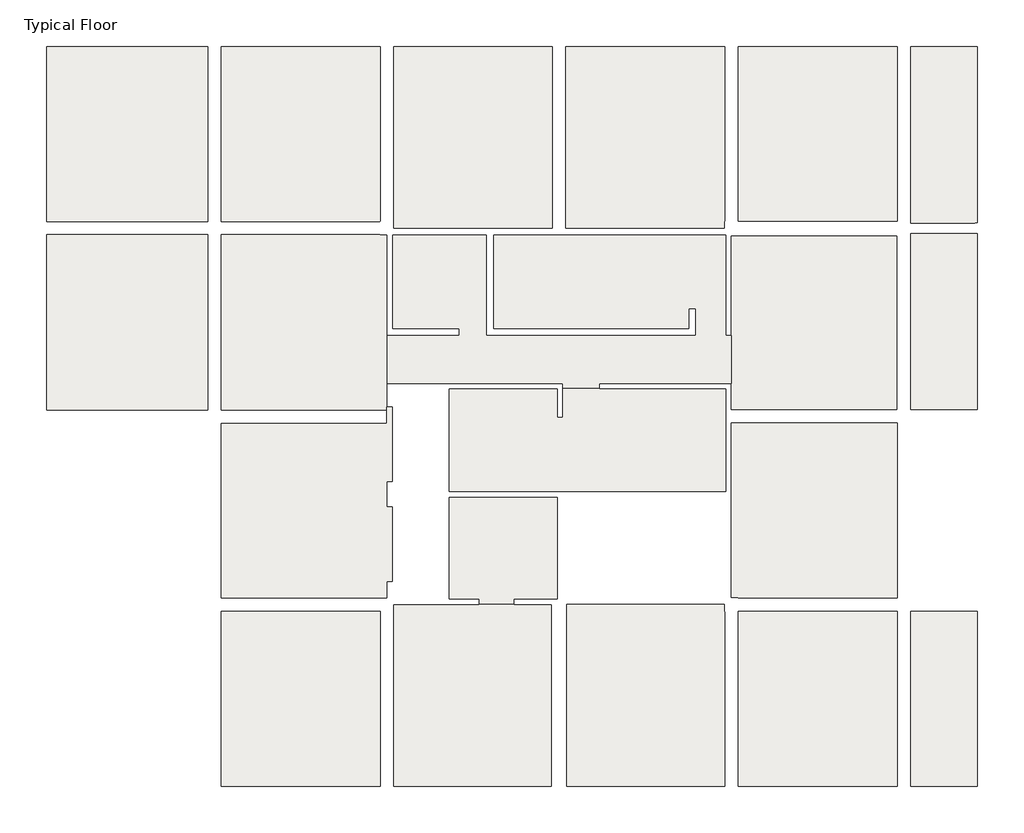
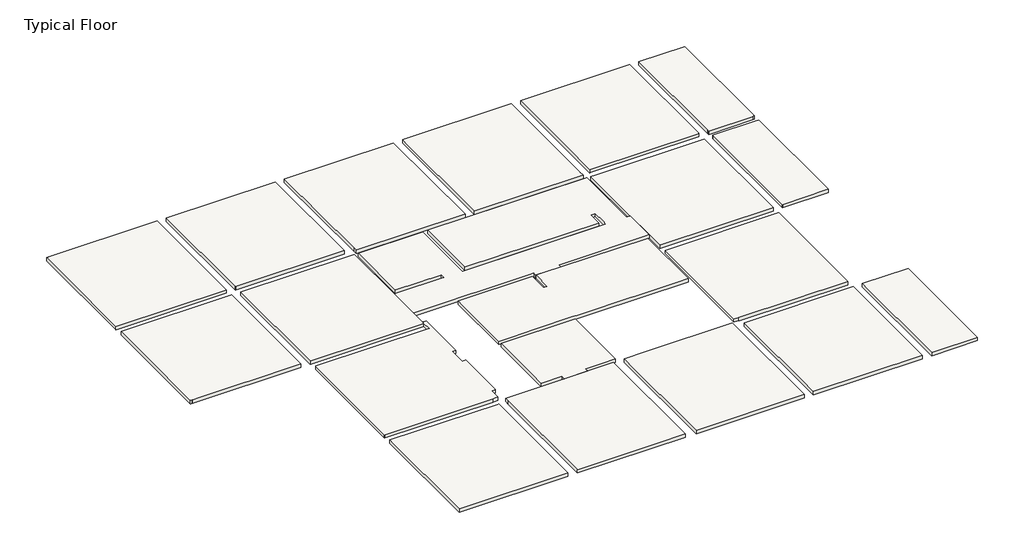
# One storey: 20 slabs.
"""IFC4 building model written with IfcOpenShell, lengths in millimetres."""

from ifc_helpers import new_model, si_unit, frame, origin, place, context, project, spatial, polyline, outline, extrude, faceted_brep, element, save

model = new_model("IFC4")

# Units and contexts
model_context = context("Model", 3, world=origin())
ifc_project = project(units=[si_unit("LENGTHUNIT", "METRE", prefix="MILLI")], contexts=[model_context])

# Site, building, storey
site = spatial("IfcSite", under=ifc_project)
building = spatial("IfcBuilding", under=site)
storey = spatial("IfcBuildingStorey", under=building, Name="Typical Floor", Elevation=4000.0)

# Slabs
placement = place(None, origin())
element("IfcSlab", 1, ObjectType="23", at=placement, inside=storey, context=model_context, shape_type="Brep", body=[
    faceted_brep([(8756.9599651, 6086.2983934, 3770.0), (-3356.6009397, 6086.2983934, 3770.0), (-3356.6009397, 10573.3383922, 3770.0), (1372.1290873, 10573.3383922, 3770.0), (1372.1290873, 9338.5905192, 3770.0), (1622.1290873, 9338.5905192, 3770.0), (1622.1290873, 10573.3383922, 3770.0), (1622.1290873, 10593.3383922, 3770.0), (3208.0390271, 10593.3383922, 3770.0), (3208.0390271, 10573.3383922, 3770.0), (8756.9599651, 10573.3383922, 3770.0), (-3356.6009397, 6086.2983934, 4000.0), (1378.3544453, 6086.2983934, 4000.0), (1628.3544453, 6086.2983934, 4000.0), (8756.9599651, 6086.2983934, 4000.0), (8756.9599651, 10573.3383922, 4000.0), (3208.0390271, 10573.3383922, 4000.0), (3208.0390271, 10593.3383922, 4000.0), (1622.1290873, 10593.3383922, 4000.0), (1622.1290873, 10573.3383922, 4000.0), (1622.1290873, 9338.5905192, 4000.0), (1372.1290873, 9338.5905192, 4000.0), (1372.1290873, 10573.3383922, 4000.0), (-3356.6009397, 10573.3383922, 4000.0)], [[[0, 1, 2, 3, 4, 5, 6, 7, 8, 9, 10]], [[11, 12, 13, 14, 15, 16, 17, 18, 19, 20, 21, 22, 23]], [[1, 0, 14, 13, 12, 11]], [[2, 1, 11, 23]], [[3, 2, 23, 22]], [[4, 3, 22, 21]], [[5, 4, 21, 20]], [[5, 20, 19, 18, 7, 6]], [[8, 7, 18, 17]], [[9, 8, 17, 16]], [[10, 9, 16, 15]], [[0, 10, 15, 14]]]),
])
element("IfcSlab", 2, ObjectType="23", at=placement, inside=storey, context=model_context, shape_type="Brep", body=[
    faceted_brep([(9298.3595467, 17938.0356779, 3770.0), (9298.3595467, 25592.9632364, 3770.0), (9303.3595467, 25592.9632364, 3770.0), (9303.3595467, 25597.9632364, 3770.0), (16261.8802114, 25597.9632364, 3770.0), (16261.8802114, 25592.9632364, 3770.0), (16266.8802114, 25592.9632364, 3770.0), (16266.8802114, 17943.0356779, 3770.0), (16261.8802114, 17943.0356779, 3770.0), (16261.8802114, 17938.0356779, 3770.0), (9303.3595467, 17938.0356779, 3770.0), (9298.3595467, 25592.9632364, 4000.0), (9298.3595467, 17938.0356779, 4000.0), (9303.3595467, 17938.0356779, 4000.0), (16261.8802114, 17938.0356779, 4000.0), (16261.8802114, 17943.0356779, 4000.0), (16266.8802114, 17943.0356779, 4000.0), (16266.8802114, 25592.9632364, 4000.0), (16261.8802114, 25592.9632364, 4000.0), (16261.8802114, 25597.9632364, 4000.0), (9303.3595467, 25597.9632364, 4000.0), (9303.3595467, 25592.9632364, 4000.0)], [[[0, 1, 2, 3, 4, 5, 6, 7, 8, 9, 10]], [[11, 12, 13, 14, 15, 16, 17, 18, 19, 20, 21]], [[6, 17, 16, 7]], [[12, 0, 10, 9, 14, 13]], [[0, 12, 11, 1]], [[3, 20, 19, 4]], [[2, 21, 20, 3]], [[21, 2, 1, 11]], [[5, 18, 17, 6]], [[18, 5, 4, 19]], [[8, 15, 14, 9]], [[15, 8, 7, 16]]]),
])
element("IfcSlab", 3, ObjectType="23", at=placement, inside=storey, context=model_context, shape_type="Brep", body=[
    faceted_brep([(16861.8802114, 25597.9632364, 3770.0), (19788.3855721, 25597.9632364, 3770.0), (19788.3855721, 25592.9632364, 3770.0), (19788.3855721, 17886.6191558, 3770.0), (19778.3855721, 17886.6191558, 3770.0), (19678.3855721, 17886.6191558, 3770.0), (19678.3855721, 17863.0356779, 3770.0), (16861.8802114, 17863.0356779, 3770.0), (16861.8802114, 17936.6191558, 3770.0), (16861.8802114, 17943.0356779, 3770.0), (16856.8802114, 17943.0356779, 3770.0), (16856.8802114, 25592.9632364, 3770.0), (16861.8802114, 25592.9632364, 3770.0), (19788.3855721, 25597.9632364, 4000.0), (16861.8802114, 25597.9632364, 4000.0), (16861.8802114, 25592.9632364, 4000.0), (16856.8802114, 25592.9632364, 4000.0), (16856.8802114, 17943.0356779, 4000.0), (16861.8802114, 17943.0356779, 4000.0), (16861.8802114, 17863.0356779, 4000.0), (19678.3855721, 17863.0356779, 4000.0), (19678.3855721, 17886.6191558, 4000.0), (19788.3855721, 17886.6191558, 4000.0), (19788.3855721, 25592.9632364, 4000.0)], [[[0, 1, 2, 3, 4, 5, 6, 7, 8, 9, 10, 11, 12]], [[13, 14, 15, 16, 17, 18, 19, 20, 21, 22, 23]], [[1, 13, 23, 22, 3, 2]], [[19, 7, 6, 20]], [[16, 11, 10, 17]], [[13, 1, 0, 14]], [[12, 15, 14, 0]], [[15, 12, 11, 16]], [[18, 9, 8, 7, 19]], [[9, 18, 17, 10]], [[5, 21, 20, 6]], [[21, 5, 4, 3, 22]]]),
])
element("IfcSlab", 4, ObjectType="23", at=placement, inside=storey, context=model_context, shape_type="Brep", body=[
    faceted_brep([(-6424.7845121, 832.5009852, 3770.0), (-6390.1585821, 832.5009852, 3770.0), (-6385.1585821, 832.5009852, 3770.0), (-6385.1585821, -6825.0062825, 3770.0), (-6390.1585821, -6825.0062825, 3770.0), (-6390.1585821, -6830.0062825, 3770.0), (-13343.8144749, -6830.0062825, 3770.0), (-13343.8144749, -6825.0062825, 3770.0), (-13348.8144749, -6825.0062825, 3770.0), (-13348.8144749, 832.5009852, 3770.0), (-13343.8144749, 832.5009852, 3770.0), (-13343.8144749, 837.5009852, 3770.0), (-6424.7845121, 837.5009852, 3770.0), (-6385.1585821, 832.5009852, 4000.0), (-6424.7845121, 832.5009852, 4000.0), (-6424.7845121, 837.5009852, 4000.0), (-13343.8144749, 837.5009852, 4000.0), (-13343.8144749, 832.5009852, 4000.0), (-13348.8144749, 832.5009852, 4000.0), (-13348.8144749, -6825.0062825, 4000.0), (-13343.8144749, -6825.0062825, 4000.0), (-13343.8144749, -6830.0062825, 4000.0), (-6390.1585821, -6830.0062825, 4000.0), (-6390.1585821, -6825.0062825, 4000.0), (-6385.1585821, -6825.0062825, 4000.0)], [[[0, 1, 2, 3, 4, 5, 6, 7, 8, 9, 10, 11, 12]], [[13, 14, 15, 16, 17, 18, 19, 20, 21, 22, 23, 24]], [[2, 13, 24, 3]], [[21, 6, 5, 22]], [[18, 9, 8, 19]], [[15, 12, 11, 16]], [[0, 14, 13, 2, 1]], [[14, 0, 12, 15]], [[10, 17, 16, 11]], [[17, 10, 9, 18]], [[20, 7, 6, 21]], [[7, 20, 19, 8]], [[4, 23, 22, 5]], [[23, 4, 3, 24]]]),
])
element("IfcSlab", 5, ObjectType="23", at=placement, inside=storey, context=model_context, shape_type="Brep", body=[
    faceted_brep([(-5795.1585821, 832.5009852, 3770.0), (-5790.1585821, 832.5009852, 3770.0), (-5784.7845121, 832.5009852, 3770.0), (-5784.7845121, 1127.9140303, 3770.0), (-2044.60675, 1127.9140303, 3770.0), (-2044.60675, 1132.9140303, 3770.0), (-534.9574452, 1132.9140303, 3770.0), (-534.9574452, 1127.9140303, 3770.0), (1107.0810158, 1127.9140303, 3770.0), (1112.0810158, 1127.9140303, 3770.0), (1112.0810158, -6825.0062825, 3770.0), (1107.0810158, -6825.0062825, 3770.0), (1107.0810158, -6830.0062825, 3770.0), (-5790.1585821, -6830.0062825, 3770.0), (-5790.1585821, -6825.0062825, 3770.0), (-5795.1585821, -6825.0062825, 3770.0), (-5784.7845121, 832.5009852, 4000.0), (-5795.1585821, 832.5009852, 4000.0), (-5795.1585821, -6825.0062825, 4000.0), (-5790.1585821, -6825.0062825, 4000.0), (-5790.1585821, -6830.0062825, 4000.0), (1107.0810158, -6830.0062825, 4000.0), (1107.0810158, -6825.0062825, 4000.0), (1112.0810158, -6825.0062825, 4000.0), (1112.0810158, 1127.9140303, 4000.0), (-534.9574452, 1127.9140303, 4000.0), (-534.9574452, 1132.9140303, 4000.0), (-2044.60675, 1132.9140303, 4000.0), (-2044.60675, 1127.9140303, 4000.0), (-5784.7845121, 1127.9140303, 4000.0)], [[[0, 1, 2, 3, 4, 5, 6, 7, 8, 9, 10, 11, 12, 13, 14, 15]], [[16, 17, 18, 19, 20, 21, 22, 23, 24, 25, 26, 27, 28, 29]], [[23, 10, 9, 24]], [[12, 21, 20, 13]], [[17, 0, 15, 18]], [[5, 27, 26, 6]], [[2, 16, 29, 3]], [[16, 2, 1, 0, 17]], [[22, 11, 10, 23]], [[11, 22, 21, 12]], [[19, 14, 13, 20]], [[14, 19, 18, 15]], [[28, 4, 3, 29]], [[4, 28, 27, 5]], [[7, 25, 24, 9, 8]], [[25, 7, 6, 26]]]),
])
element("IfcSlab", 6, ObjectType="23", at=placement, inside=storey, context=model_context, shape_type="Brep", body=[
    faceted_brep([(8703.3595467, 812.5009852, 3770.0), (8708.3595467, 812.5009852, 3770.0), (8708.3595467, -6825.0062825, 3770.0), (8703.3595467, -6825.0062825, 3770.0), (8703.3595467, -6830.0062825, 3770.0), (1807.0810158, -6830.0062825, 3770.0), (1807.0810158, -6825.0062825, 3770.0), (1802.0810158, -6825.0062825, 3770.0), (1802.0810158, 1138.5687304, 3770.0), (1807.0810158, 1138.5687304, 3770.0), (3208.0390271, 1138.5687304, 3770.0), (3208.0390271, 1133.5687304, 3770.0), (8703.3595467, 1133.5687304, 3770.0), (8708.3595467, 812.5009852, 4000.0), (8703.3595467, 812.5009852, 4000.0), (8703.3595467, 1133.5687304, 4000.0), (3208.0390271, 1133.5687304, 4000.0), (3208.0390271, 1138.5687304, 4000.0), (1807.0810158, 1138.5687304, 4000.0), (1802.0810158, 1138.5687304, 4000.0), (1802.0810158, -6825.0062825, 4000.0), (1807.0810158, -6825.0062825, 4000.0), (1807.0810158, -6830.0062825, 4000.0), (8703.3595467, -6830.0062825, 4000.0), (8703.3595467, -6825.0062825, 4000.0), (8708.3595467, -6825.0062825, 4000.0)], [[[0, 1, 2, 3, 4, 5, 6, 7, 8, 9, 10, 11, 12]], [[13, 14, 15, 16, 17, 18, 19, 20, 21, 22, 23, 24, 25]], [[8, 19, 18, 17, 10, 9]], [[1, 13, 25, 2]], [[4, 23, 22, 5]], [[19, 8, 7, 20]], [[0, 14, 13, 1]], [[14, 0, 12, 15]], [[24, 3, 2, 25]], [[3, 24, 23, 4]], [[6, 21, 20, 7]], [[21, 6, 5, 22]], [[11, 16, 15, 12]], [[16, 11, 10, 17]]]),
])
element("IfcSlab", 7, ObjectType="23", at=placement, inside=storey, context=model_context, shape_type="Brep", body=[
    faceted_brep([(16261.8802114, 832.5009852, 3770.0), (16266.8802114, 832.5009852, 3770.0), (16266.8802114, -6825.0062825, 3770.0), (16261.8802114, -6825.0062825, 3770.0), (16261.8802114, -6830.0062825, 3770.0), (9303.3595467, -6830.0062825, 3770.0), (9303.3595467, -6825.0062825, 3770.0), (9298.3595467, -6825.0062825, 3770.0), (9298.3595467, 812.5009852, 3770.0), (9303.3595467, 812.5009852, 3770.0), (9303.3595467, 832.5009852, 3770.0), (9303.3595467, 837.5009852, 3770.0), (16261.8802114, 837.5009852, 3770.0), (16266.8802114, 832.5009852, 4000.0), (16261.8802114, 832.5009852, 4000.0), (16261.8802114, 837.5009852, 4000.0), (9303.3595467, 837.5009852, 4000.0), (9303.3595467, 812.5009852, 4000.0), (9298.3595467, 812.5009852, 4000.0), (9298.3595467, -6825.0062825, 4000.0), (9303.3595467, -6825.0062825, 4000.0), (9303.3595467, -6830.0062825, 4000.0), (16261.8802114, -6830.0062825, 4000.0), (16261.8802114, -6825.0062825, 4000.0), (16266.8802114, -6825.0062825, 4000.0)], [[[0, 1, 2, 3, 4, 5, 6, 7, 8, 9, 10, 11, 12]], [[13, 14, 15, 16, 17, 18, 19, 20, 21, 22, 23, 24]], [[15, 12, 11, 16]], [[1, 13, 24, 2]], [[21, 5, 4, 22]], [[18, 8, 7, 19]], [[0, 14, 13, 1]], [[14, 0, 12, 15]], [[9, 17, 16, 11, 10]], [[17, 9, 8, 18]], [[6, 20, 19, 7]], [[20, 6, 5, 21]], [[23, 3, 2, 24]], [[3, 23, 22, 4]]]),
])
element("IfcSlab", 8, ObjectType="23", at=placement, inside=storey, context=model_context, shape_type="Brep", body=[
    faceted_brep([(19786.5095237, 837.5009852, 3770.0), (19786.5074854, 832.5009852, 3770.0), (19783.3837564, -6830.0062825, 3770.0), (19778.383756, -6830.0062825, 3770.0), (16861.8802114, -6830.0062825, 3770.0), (16861.8802114, -6825.0062825, 3770.0), (16856.8802114, -6825.0062825, 3770.0), (16856.8802114, 832.5009852, 3770.0), (16861.8802114, 832.5009852, 3770.0), (16861.8802114, 837.5009852, 3770.0), (19783.3837564, -6830.0062825, 4000.0), (19786.5074854, 832.5009852, 4000.0), (19786.5095237, 837.5009852, 4000.0), (16861.8802114, 837.5009852, 4000.0), (16861.8802114, 832.5009852, 4000.0), (16856.8802114, 832.5009852, 4000.0), (16856.8802114, -6825.0062825, 4000.0), (16861.8802114, -6825.0062825, 4000.0), (16861.8802114, -6830.0062825, 4000.0), (19778.383756, -6830.0062825, 4000.0)], [[[0, 1, 2, 3, 4, 5, 6, 7, 8, 9]], [[10, 11, 12, 13, 14, 15, 16, 17, 18, 19]], [[2, 1, 0, 12, 11, 10]], [[2, 10, 19, 18, 4, 3]], [[15, 7, 6, 16]], [[12, 0, 9, 13]], [[8, 14, 13, 9]], [[14, 8, 7, 15]], [[5, 17, 16, 6]], [[17, 5, 4, 18]]]),
])
element("IfcSlab", 9, ObjectType="23", at=placement, inside=storey, context=model_context, shape_type="SweptSolid", body=[
    extrude(outline(polyline([(1378.3544453, 5836.2983934), (1378.3544453, 1377.9140303), (-534.9574452, 1377.9140303), (-534.9574452, 1132.9140303), (-2044.60675, 1132.9140303), (-2044.60675, 1377.9140303), (-3356.6009397, 1377.9140303), (-3356.6009397, 5836.2983934), (1378.3544453, 5836.2983934)])), frame((0.0, 0.0, 3770.0), z_axis=(0.0, 0.0, 1.0), x_axis=(1.0, 0.0, 0.0)), (0.0, 0.0, 1.0), 230.0),
])
element("IfcSlab", 10, ObjectType="23", at=placement, inside=storey, context=model_context, shape_type="Brep", body=[
    faceted_brep([(-6090.1585821, 9071.6131842, 3770.0), (-6090.1585821, 9661.6131842, 3770.0), (-6090.1585821, 9666.6131842, 3770.0), (-6090.1585821, 9791.4853106, 3770.0), (-5844.2021017, 9791.4853106, 3770.0), (-5844.2021017, 6520.0597037, 3770.0), (-6094.2021017, 6520.0597037, 3770.0), (-6094.2021017, 5411.9459871, 3770.0), (-5844.2021017, 5411.9459871, 3770.0), (-5844.2021017, 2140.5203801, 3770.0), (-5898.8711202, 2140.5203801, 3770.0), (-6098.8711202, 2140.5203801, 3770.0), (-6098.8711202, 1432.5009852, 3770.0), (-6424.7845121, 1432.5009852, 3770.0), (-6424.7845121, 1430.5203801, 3770.0), (-13343.8144749, 1430.5203801, 3770.0), (-13343.8144749, 1432.5009852, 3770.0), (-13348.8144749, 1432.5009852, 3770.0), (-13348.8144749, 9066.6131842, 3770.0), (-13343.8144749, 9066.6131842, 3770.0), (-13343.8144749, 9071.6131842, 3770.0), (-6090.1585821, 9666.6131842, 4000.0), (-6090.1585821, 9661.6131842, 4000.0), (-6090.1585821, 9071.6131842, 4000.0), (-13343.8144749, 9071.6131842, 4000.0), (-13343.8144749, 9066.6131842, 4000.0), (-13348.8144749, 9066.6131842, 4000.0), (-13348.8144749, 1432.5009852, 4000.0), (-13343.8144749, 1432.5009852, 4000.0), (-13343.8144749, 1430.5203801, 4000.0), (-6424.7845121, 1430.5203801, 4000.0), (-6424.7845121, 1432.5009852, 4000.0), (-6098.8711202, 1432.5009852, 4000.0), (-6098.8711202, 2140.5203801, 4000.0), (-5898.8711202, 2140.5203801, 4000.0), (-5844.2021017, 2140.5203801, 4000.0), (-5844.2021017, 5411.9459871, 4000.0), (-6094.2021017, 5411.9459871, 4000.0), (-6094.2021017, 6520.0597037, 4000.0), (-5844.2021017, 6520.0597037, 4000.0), (-5844.2021017, 9791.4853106, 4000.0), (-6090.1585821, 9791.4853106, 4000.0)], [[[0, 1, 2, 3, 4, 5, 6, 7, 8, 9, 10, 11, 12, 13, 14, 15, 16, 17, 18, 19, 20]], [[21, 22, 23, 24, 25, 26, 27, 28, 29, 30, 31, 32, 33, 34, 35, 36, 37, 38, 39, 40, 41]], [[2, 1, 0, 23, 22, 21]], [[3, 2, 21, 41]], [[4, 3, 41, 40]], [[5, 4, 40, 39]], [[6, 5, 39, 38]], [[7, 6, 38, 37]], [[8, 7, 37, 36]], [[9, 8, 36, 35]], [[9, 35, 34, 33, 11, 10]], [[11, 33, 32, 12]], [[29, 15, 14, 30]], [[26, 18, 17, 27]], [[23, 0, 20, 24]], [[19, 25, 24, 20]], [[25, 19, 18, 26]], [[28, 16, 15, 29]], [[16, 28, 27, 17]], [[13, 31, 30, 14]], [[31, 13, 12, 32]]]),
])
element("IfcSlab", 11, ObjectType="23", at=placement, inside=storey, context=model_context, shape_type="Brep", body=[
    faceted_brep([(-13943.8144749, 17336.6191558, 3770.0), (-13938.8144749, 17336.6191558, 3770.0), (-13938.8144749, 9666.6131842, 3770.0), (-13943.8144749, 9666.6131842, 3770.0), (-13943.8144749, 9661.6131842, 3770.0), (-20894.7160223, 9661.6131842, 3770.0), (-20894.7160223, 9666.6131842, 3770.0), (-20994.7160223, 9666.6131842, 3770.0), (-20999.7160223, 9666.6131842, 3770.0), (-20999.7160223, 17336.6191558, 3770.0), (-20994.7160223, 17336.6191558, 3770.0), (-20994.7160223, 17341.6191558, 3770.0), (-13943.8144749, 17341.6191558, 3770.0), (-13938.8144749, 17336.6191558, 4000.0), (-13943.8144749, 17336.6191558, 4000.0), (-13943.8144749, 17341.6191558, 4000.0), (-20994.7160223, 17341.6191558, 4000.0), (-20994.7160223, 17336.6191558, 4000.0), (-20999.7160223, 17336.6191558, 4000.0), (-20999.7160223, 9666.6131842, 4000.0), (-20894.7160223, 9666.6131842, 4000.0), (-20894.7160223, 9661.6131842, 4000.0), (-13943.8144749, 9661.6131842, 4000.0), (-13943.8144749, 9666.6131842, 4000.0), (-13938.8144749, 9666.6131842, 4000.0)], [[[0, 1, 2, 3, 4, 5, 6, 7, 8, 9, 10, 11, 12]], [[13, 14, 15, 16, 17, 18, 19, 20, 21, 22, 23, 24]], [[1, 13, 24, 2]], [[4, 22, 21, 5]], [[8, 19, 18, 9]], [[15, 12, 11, 16]], [[0, 14, 13, 1]], [[14, 0, 12, 15]], [[3, 23, 22, 4]], [[23, 3, 2, 24]], [[6, 20, 19, 8, 7]], [[20, 6, 5, 21]], [[10, 17, 16, 11]], [[17, 10, 9, 18]]]),
])
element("IfcSlab", 12, ObjectType="23", at=placement, inside=storey, context=model_context, shape_type="Brep", body=[
    faceted_brep([(-6090.1585821, 9791.4853106, 3770.0), (-6090.1585821, 9666.6131842, 3770.0), (-6090.1585821, 9661.6131842, 3770.0), (-13343.8144749, 9661.6131842, 3770.0), (-13343.8144749, 9666.6131842, 3770.0), (-13348.8144749, 9666.6131842, 3770.0), (-13348.8144749, 17336.6191558, 3770.0), (-13343.8144749, 17336.6191558, 3770.0), (-13343.8144749, 17341.6191558, 3770.0), (-6390.1585821, 17341.6191558, 3770.0), (-6390.1585821, 17336.6191558, 3770.0), (-6090.1585821, 17336.6191558, 3770.0), (-6090.1585821, 12927.509382, 3770.0), (-6084.2021017, 12927.509382, 3770.0), (-6084.2021017, 10823.3383922, 3770.0), (-6094.2021017, 10823.3383922, 3770.0), (-6094.2021017, 9791.4853106, 3770.0), (-6090.1585821, 9666.6131842, 4000.0), (-6090.1585821, 9791.4853106, 4000.0), (-6094.2021017, 9791.4853106, 4000.0), (-6094.2021017, 10573.3383922, 4000.0), (-6094.2021017, 10823.3383922, 4000.0), (-6084.2021017, 10823.3383922, 4000.0), (-6084.2021017, 12927.509382, 4000.0), (-6090.1585821, 12927.509382, 4000.0), (-6090.1585821, 17336.6191558, 4000.0), (-6390.1585821, 17336.6191558, 4000.0), (-6390.1585821, 17341.6191558, 4000.0), (-13343.8144749, 17341.6191558, 4000.0), (-13343.8144749, 17336.6191558, 4000.0), (-13348.8144749, 17336.6191558, 4000.0), (-13348.8144749, 9666.6131842, 4000.0), (-13343.8144749, 9666.6131842, 4000.0), (-13343.8144749, 9661.6131842, 4000.0), (-6090.1585821, 9661.6131842, 4000.0)], [[[0, 1, 2, 3, 4, 5, 6, 7, 8, 9, 10, 11, 12, 13, 14, 15, 16]], [[17, 18, 19, 20, 21, 22, 23, 24, 25, 26, 27, 28, 29, 30, 31, 32, 33, 34]], [[13, 23, 22, 14]], [[2, 34, 33, 3]], [[30, 6, 5, 31]], [[27, 9, 8, 28]], [[10, 26, 25, 11]], [[26, 10, 9, 27]], [[1, 17, 34, 2]], [[17, 1, 0, 18]], [[7, 29, 28, 8]], [[29, 7, 6, 30]], [[32, 4, 3, 33]], [[4, 32, 31, 5]], [[24, 12, 11, 25]], [[12, 24, 23, 13]], [[21, 15, 14, 22]], [[15, 21, 20, 19, 16]], [[16, 19, 18, 0]]]),
])
element("IfcSlab", 13, ObjectType="23", at=placement, inside=storey, context=model_context, shape_type="SweptSolid", body=[
    extrude(outline(polyline([(-6390.1585821, 25592.9632364), (-6385.1585821, 25592.9632364), (-6385.1585821, 17936.6191558), (-6390.1585821, 17936.6191558), (-6390.1585821, 17931.6191558), (-13343.8144749, 17931.6191558), (-13343.8144749, 17936.6191558), (-13348.8144749, 17936.6191558), (-13348.8144749, 25592.9632364), (-13343.8144749, 25592.9632364), (-13343.8144749, 25597.9632364), (-6390.1585821, 25597.9632364), (-6390.1585821, 25592.9632364)])), frame((0.0, 0.0, 3770.0), z_axis=(0.0, 0.0, 1.0), x_axis=(1.0, 0.0, 0.0)), (0.0, 0.0, 1.0), 230.0),
])
element("IfcSlab", 14, ObjectType="23", at=placement, inside=storey, context=model_context, shape_type="Brep", body=[
    faceted_brep([(-13943.8144749, 17936.6191558, 3770.0), (-13943.8144749, 17931.6191558, 3770.0), (-20994.7160223, 17931.6191558, 3770.0), (-20994.7160223, 17936.6191558, 3770.0), (-20999.7160223, 17936.6191558, 3770.0), (-20999.7160223, 25592.9632364, 3770.0), (-20994.7160223, 25592.9632364, 3770.0), (-20894.7160223, 25592.9632364, 3770.0), (-20894.7160223, 25597.9632364, 3770.0), (-13943.8144749, 25597.9632364, 3770.0), (-13943.8144749, 25592.9632364, 3770.0), (-13938.8144749, 25592.9632364, 3770.0), (-13938.8144749, 17936.6191558, 3770.0), (-13943.8144749, 17931.6191558, 4000.0), (-13943.8144749, 17936.6191558, 4000.0), (-13938.8144749, 17936.6191558, 4000.0), (-13938.8144749, 25592.9632364, 4000.0), (-13943.8144749, 25592.9632364, 4000.0), (-13943.8144749, 25597.9632364, 4000.0), (-20894.7160223, 25597.9632364, 4000.0), (-20894.7160223, 25592.9632364, 4000.0), (-20999.7160223, 25592.9632364, 4000.0), (-20999.7160223, 17936.6191558, 4000.0), (-20994.7160223, 17936.6191558, 4000.0), (-20994.7160223, 17931.6191558, 4000.0)], [[[0, 1, 2, 3, 4, 5, 6, 7, 8, 9, 10, 11, 12]], [[13, 14, 15, 16, 17, 18, 19, 20, 21, 22, 23, 24]], [[15, 12, 11, 16]], [[1, 13, 24, 2]], [[21, 5, 4, 22]], [[18, 9, 8, 19]], [[0, 14, 13, 1]], [[14, 0, 12, 15]], [[10, 17, 16, 11]], [[17, 10, 9, 18]], [[7, 20, 19, 8]], [[20, 7, 6, 5, 21]], [[3, 23, 22, 4]], [[23, 3, 2, 24]]]),
])
element("IfcSlab", 15, ObjectType="23", at=placement, inside=storey, context=model_context, shape_type="Brep", body=[
    faceted_brep([(-5790.1585821, 25592.9632364, 3770.0), (-5790.1585821, 25597.9632364, 3770.0), (1157.0810158, 25597.9632364, 3770.0), (1157.0810158, 25592.9632364, 3770.0), (1162.0810158, 25592.9632364, 3770.0), (1162.0810158, 17636.6191558, 3770.0), (1157.0810158, 17636.6191558, 3770.0), (-5790.1585821, 17636.6191558, 3770.0), (-5790.1585821, 17936.6191558, 3770.0), (-5795.1585821, 17936.6191558, 3770.0), (-5795.1585821, 25592.9632364, 3770.0), (-5790.1585821, 25597.9632364, 4000.0), (-5790.1585821, 25592.9632364, 4000.0), (-5795.1585821, 25592.9632364, 4000.0), (-5795.1585821, 17936.6191558, 4000.0), (-5790.1585821, 17936.6191558, 4000.0), (-5790.1585821, 17636.6191558, 4000.0), (1162.0810158, 17636.6191558, 4000.0), (1162.0810158, 25592.9632364, 4000.0), (1157.0810158, 25592.9632364, 4000.0), (1157.0810158, 25597.9632364, 4000.0)], [[[0, 1, 2, 3, 4, 5, 6, 7, 8, 9, 10]], [[11, 12, 13, 14, 15, 16, 17, 18, 19, 20]], [[4, 18, 17, 5]], [[13, 10, 9, 14]], [[1, 11, 20, 2]], [[0, 12, 11, 1]], [[12, 0, 10, 13]], [[8, 15, 14, 9]], [[15, 8, 7, 16]], [[3, 19, 18, 4]], [[19, 3, 2, 20]], [[7, 6, 5, 17, 16]]]),
])
element("IfcSlab", 16, ObjectType="23", at=placement, inside=storey, context=model_context, shape_type="Brep", body=[
    faceted_brep([(1757.0810158, 25592.9632364, 3770.0), (1757.0810158, 25597.9632364, 3770.0), (8703.3595467, 25597.9632364, 3770.0), (8703.3595467, 25592.9632364, 3770.0), (8708.3595467, 25592.9632364, 3770.0), (8708.3595467, 17936.6191558, 3770.0), (8703.3595467, 17936.6191558, 3770.0), (8703.3595467, 17636.6191558, 3770.0), (1757.0810158, 17636.6191558, 3770.0), (1752.0810158, 17636.6191558, 3770.0), (1752.0810158, 25592.9632364, 3770.0), (1757.0810158, 25597.9632364, 4000.0), (1757.0810158, 25592.9632364, 4000.0), (1752.0810158, 25592.9632364, 4000.0), (1752.0810158, 17636.6191558, 4000.0), (8703.3595467, 17636.6191558, 4000.0), (8703.3595467, 17936.6191558, 4000.0), (8708.3595467, 17936.6191558, 4000.0), (8708.3595467, 25592.9632364, 4000.0), (8703.3595467, 25592.9632364, 4000.0), (8703.3595467, 25597.9632364, 4000.0)], [[[0, 1, 2, 3, 4, 5, 6, 7, 8, 9, 10]], [[11, 12, 13, 14, 15, 16, 17, 18, 19, 20]], [[17, 5, 4, 18]], [[13, 10, 9, 14]], [[1, 11, 20, 2]], [[0, 12, 11, 1]], [[12, 0, 10, 13]], [[6, 16, 15, 7]], [[16, 6, 5, 17]], [[3, 19, 18, 4]], [[19, 3, 2, 20]], [[9, 8, 7, 15, 14]]]),
])
element("IfcSlab", 17, ObjectType="23", at=placement, inside=storey, context=model_context, shape_type="Brep", body=[
    faceted_brep([(16861.8802114, 17343.0356779, 3770.0), (16861.8802114, 17396.6191558, 3770.0), (19678.3855721, 17396.6191558, 3770.0), (19678.3855721, 17386.6191558, 3770.0), (19778.3855721, 17386.6191558, 3770.0), (19788.3855721, 17386.6191558, 3770.0), (19788.3855721, 17336.6191558, 3770.0), (19788.3855721, 9676.6131842, 3770.0), (19778.3855721, 9676.6131842, 3770.0), (16861.8802114, 9676.6131842, 3770.0), (16861.8802114, 9681.6131842, 3770.0), (16856.8802114, 9681.6131842, 3770.0), (16856.8802114, 17293.0356779, 3770.0), (16856.8802114, 17343.0356779, 3770.0), (16861.8802114, 17396.6191558, 4000.0), (16861.8802114, 17343.0356779, 4000.0), (16856.8802114, 17343.0356779, 4000.0), (16856.8802114, 17293.0356779, 4000.0), (16856.8802114, 9681.6131842, 4000.0), (16861.8802114, 9681.6131842, 4000.0), (16861.8802114, 9676.6131842, 4000.0), (19778.3855721, 9676.6131842, 4000.0), (19788.3855721, 9676.6131842, 4000.0), (19788.3855721, 17336.6191558, 4000.0), (19788.3855721, 17386.6191558, 4000.0), (19678.3855721, 17386.6191558, 4000.0), (19678.3855721, 17396.6191558, 4000.0)], [[[0, 1, 2, 3, 4, 5, 6, 7, 8, 9, 10, 11, 12, 13]], [[14, 15, 16, 17, 18, 19, 20, 21, 22, 23, 24, 25, 26]], [[1, 14, 26, 2]], [[22, 7, 6, 5, 24, 23]], [[7, 22, 21, 20, 9, 8]], [[16, 13, 12, 11, 18, 17]], [[0, 15, 14, 1]], [[15, 0, 13, 16]], [[19, 10, 9, 20]], [[10, 19, 18, 11]], [[3, 25, 24, 5, 4]], [[25, 3, 2, 26]]]),
])
element("IfcSlab", 18, ObjectType="23", at=placement, inside=storey, context=model_context, shape_type="Brep", body=[
    faceted_brep([(16261.8802114, 17293.0356779, 3770.0), (16261.8802114, 9681.6131842, 3770.0), (9006.9599651, 9681.6131842, 3770.0), (9006.9599651, 10823.3383922, 3770.0), (9003.3595467, 10823.3383922, 3770.0), (9003.3595467, 12927.509382, 3770.0), (9006.9599651, 12927.509382, 3770.0), (9006.9599651, 17293.0356779, 3770.0), (16261.8802114, 9681.6131842, 4000.0), (16261.8802114, 17293.0356779, 4000.0), (9303.3595467, 17293.0356779, 4000.0), (9006.9599651, 17293.0356779, 4000.0), (9006.9599651, 12927.509382, 4000.0), (9003.3595467, 12927.509382, 4000.0), (9003.3595467, 10823.3383922, 4000.0), (9006.9599651, 10823.3383922, 4000.0), (9006.9599651, 9681.6131842, 4000.0)], [[[0, 1, 2, 3, 4, 5, 6, 7]], [[8, 9, 10, 11, 12, 13, 14, 15, 16]], [[9, 0, 7, 11, 10]], [[1, 0, 9, 8]], [[1, 8, 16, 2]], [[13, 5, 4, 14]], [[6, 12, 11, 7]], [[12, 6, 5, 13]], [[15, 3, 2, 16]], [[3, 15, 14, 4]]]),
])
element("IfcSlab", 19, ObjectType="23", at=placement, inside=storey, context=model_context, shape_type="Brep", body=[
    faceted_brep([(9303.3595467, 1452.5009852, 3770.0), (9001.9599651, 1452.5009852, 3770.0), (9001.9599651, 1457.2873442, 3770.0), (9006.9599651, 1457.2873442, 3770.0), (9006.9599651, 9081.6131842, 3770.0), (9006.9599651, 9086.6131842, 3770.0), (16261.8802114, 9086.6131842, 3770.0), (16261.8802114, 9081.6131842, 3770.0), (16266.8802114, 9081.6131842, 3770.0), (16266.8802114, 1432.5009852, 3770.0), (16261.8802114, 1432.5009852, 3770.0), (16261.8802114, 1427.5009852, 3770.0), (9303.3595467, 1427.5009852, 3770.0), (9303.3595467, 1432.5009852, 3770.0), (9001.9599651, 1452.5009852, 4000.0), (9303.3595467, 1452.5009852, 4000.0), (9303.3595467, 1427.5009852, 4000.0), (16261.8802114, 1427.5009852, 4000.0), (16261.8802114, 1432.5009852, 4000.0), (16266.8802114, 1432.5009852, 4000.0), (16266.8802114, 9081.6131842, 4000.0), (16261.8802114, 9081.6131842, 4000.0), (16261.8802114, 9086.6131842, 4000.0), (9006.9599651, 9086.6131842, 4000.0), (9006.9599651, 1457.2873442, 4000.0), (9001.9599651, 1457.2873442, 4000.0)], [[[0, 1, 2, 3, 4, 5, 6, 7, 8, 9, 10, 11, 12, 13]], [[14, 15, 16, 17, 18, 19, 20, 21, 22, 23, 24, 25]], [[8, 20, 19, 9]], [[16, 12, 11, 17]], [[1, 14, 25, 2]], [[22, 6, 5, 23]], [[0, 15, 14, 1]], [[15, 0, 13, 12, 16]], [[7, 21, 20, 8]], [[21, 7, 6, 22]], [[18, 10, 9, 19]], [[10, 18, 17, 11]], [[3, 24, 23, 5, 4]], [[24, 3, 2, 25]]]),
])
element("IfcSlab", 20, ObjectType="23", at=placement, inside=storey, context=model_context, shape_type="Brep", body=[
    faceted_brep([(-2917.7132036, 12927.509382, 3770.0), (-2917.7132036, 13227.509382, 3770.0), (-5840.1585821, 13227.509382, 3770.0), (-5840.1585821, 17336.6191558, 3770.0), (-1734.8951916, 17336.6191558, 3770.0), (-1734.8951916, 13227.509382, 3770.0), (-1734.8951916, 12927.509382, 3770.0), (7445.9514571, 12927.509382, 3770.0), (7445.9514571, 13227.509382, 3770.0), (7445.9514571, 14114.9964125, 3770.0), (7145.9514571, 14114.9964125, 3770.0), (7145.9514571, 13227.509382, 3770.0), (-1404.8951916, 13227.509382, 3770.0), (-1404.8951916, 17336.6191558, 3770.0), (8703.3595467, 17336.6191558, 3770.0), (8756.9599651, 17336.6191558, 3770.0), (8756.9599651, 17293.0356779, 3770.0), (8756.9599651, 12927.509382, 3770.0), (9003.3595467, 12927.509382, 3770.0), (9003.3595467, 10823.3383922, 3770.0), (8756.9599651, 10823.3383922, 3770.0), (3208.0390271, 10823.3383922, 3770.0), (3208.0390271, 10593.3383922, 3770.0), (1622.1290873, 10593.3383922, 3770.0), (1622.1290873, 10823.3383922, 3770.0), (-6084.2021017, 10823.3383922, 3770.0), (-6084.2021017, 12927.509382, 3770.0), (-5840.1585821, 12927.509382, 3770.0), (-2917.7132036, 13227.509382, 4000.0), (-2917.7132036, 12927.509382, 4000.0), (-5840.1585821, 12927.509382, 4000.0), (-6084.2021017, 12927.509382, 4000.0), (-6084.2021017, 10823.3383922, 4000.0), (1622.1290873, 10823.3383922, 4000.0), (1622.1290873, 10593.3383922, 4000.0), (3208.0390271, 10593.3383922, 4000.0), (3208.0390271, 10823.3383922, 4000.0), (8756.9599651, 10823.3383922, 4000.0), (9003.3595467, 10823.3383922, 4000.0), (9003.3595467, 12927.509382, 4000.0), (8756.9599651, 12927.509382, 4000.0), (8756.9599651, 17336.6191558, 4000.0), (8703.3595467, 17336.6191558, 4000.0), (-1404.8951916, 17336.6191558, 4000.0), (-1404.8951916, 13227.509382, 4000.0), (7145.9514571, 13227.509382, 4000.0), (7145.9514571, 14114.9964125, 4000.0), (7445.9514571, 14114.9964125, 4000.0), (7445.9514571, 13227.509382, 4000.0), (7445.9514571, 12927.509382, 4000.0), (-1734.8951916, 12927.509382, 4000.0), (-1734.8951916, 13227.509382, 4000.0), (-1734.8951916, 17336.6191558, 4000.0), (-5790.1585821, 17336.6191558, 4000.0), (-5840.1585821, 17336.6191558, 4000.0), (-5840.1585821, 13227.509382, 4000.0)], [[[0, 1, 2, 3, 4, 5, 6, 7, 8, 9, 10, 11, 12, 13, 14, 15, 16, 17, 18, 19, 20, 21, 22, 23, 24, 25, 26, 27]], [[28, 29, 30, 31, 32, 33, 34, 35, 36, 37, 38, 39, 40, 41, 42, 43, 44, 45, 46, 47, 48, 49, 50, 51, 52, 53, 54, 55]], [[29, 0, 27, 26, 31, 30]], [[1, 0, 29, 28]], [[2, 1, 28, 55]], [[3, 2, 55, 54]], [[4, 3, 54, 53, 52]], [[4, 52, 51, 50, 6, 5]], [[7, 6, 50, 49]], [[7, 49, 48, 47, 9, 8]], [[10, 9, 47, 46]], [[11, 10, 46, 45]], [[12, 11, 45, 44]], [[13, 12, 44, 43]], [[15, 14, 13, 43, 42, 41]], [[17, 16, 15, 41, 40]], [[17, 40, 39, 18]], [[36, 21, 20, 19, 38, 37]], [[22, 21, 36, 35]], [[23, 22, 35, 34]], [[24, 23, 34, 33]], [[24, 33, 32, 25]], [[26, 25, 32, 31]], [[19, 18, 39, 38]]]),
])

save(model, "model.ifc")

# Revit data of these elements
# Type "23"
#   Function = 0
#   Layers, outside or top first: 23 cm "Concrete" (function 1)
# Element 1 (IfcSlab, "23")
#   Mark = "S1"
#   SOFiSTiK_AMG_Comments = ""
#   Height Offset From Level = 0 cm
#   built-in parameter 1001954 = 1
#   SOFiSTiK_AMG_Scheduled = yes
#   SOFiSTiK_AMG_Adjusted = yes
#   Phase Created = New Construction
#   Materials on its faces: "Concrete"
# Element 2 (IfcSlab, "23")
#   Mark = "S2"
#   SOFiSTiK_AMG_Comments = ""
#   Height Offset From Level = 0 cm
#   built-in parameter 1001954 = 1
#   SOFiSTiK_AMG_Scheduled = yes
#   SOFiSTiK_AMG_Adjusted = yes
#   Phase Created = New Construction
#   Materials on its faces: "Concrete"
# Element 3 (IfcSlab, "23")
#   Mark = "S3"
#   SOFiSTiK_AMG_Comments = ""
#   Height Offset From Level = 0 cm
#   built-in parameter 1001954 = 1
#   SOFiSTiK_AMG_Scheduled = yes
#   SOFiSTiK_AMG_Adjusted = yes
#   Phase Created = New Construction
#   Materials on its faces: "Concrete"
# Element 4 (IfcSlab, "23")
#   Mark = "S4"
#   SOFiSTiK_AMG_Comments = ""
#   Height Offset From Level = 0 cm
#   built-in parameter 1001954 = 1
#   SOFiSTiK_AMG_Scheduled = yes
#   SOFiSTiK_AMG_Adjusted = yes
#   Phase Created = New Construction
#   Materials on its faces: "Concrete"
# Element 5 (IfcSlab, "23")
#   Mark = "S5"
#   SOFiSTiK_AMG_Comments = ""
#   Height Offset From Level = 0 cm
#   built-in parameter 1001954 = 1
#   SOFiSTiK_AMG_Scheduled = yes
#   SOFiSTiK_AMG_Adjusted = yes
#   Phase Created = New Construction
#   Materials on its faces: "Concrete"
# Element 6 (IfcSlab, "23")
#   Mark = "S6"
#   SOFiSTiK_AMG_Comments = ""
#   built-in parameter 1001955 = 3.14159 (stored number, unit not read)
#   Height Offset From Level = 0 cm
#   built-in parameter 1001954 = 1
#   SOFiSTiK_AMG_Scheduled = yes
#   SOFiSTiK_AMG_Adjusted = yes
#   Phase Created = New Construction
#   Materials on its faces: "Concrete"
# Element 7 (IfcSlab, "23")
#   Mark = "S7"
#   SOFiSTiK_AMG_Comments = ""
#   built-in parameter 1001955 = 3.14159 (stored number, unit not read)
#   Height Offset From Level = 0 cm
#   built-in parameter 1001954 = 1
#   SOFiSTiK_AMG_Scheduled = yes
#   SOFiSTiK_AMG_Adjusted = yes
#   Phase Created = New Construction
#   Materials on its faces: "Concrete"
# Element 8 (IfcSlab, "23")
#   Mark = "S8"
#   SOFiSTiK_AMG_Comments = ""
#   Height Offset From Level = 0 cm
#   built-in parameter 1001954 = 1
#   SOFiSTiK_AMG_Scheduled = yes
#   SOFiSTiK_AMG_Adjusted = yes
#   Phase Created = New Construction
#   Materials on its faces: "Concrete"
# Element 9 (IfcSlab, "23")
#   Mark = "S9"
#   SOFiSTiK_AMG_Comments = ""
#   Height Offset From Level = 0 cm
#   built-in parameter 1001954 = 1
#   SOFiSTiK_AMG_Scheduled = yes
#   SOFiSTiK_AMG_Adjusted = yes
#   Phase Created = New Construction
#   Materials on its faces: "Concrete"
# Element 10 (IfcSlab, "23")
#   Mark = "S10"
#   SOFiSTiK_AMG_Comments = ""
#   Height Offset From Level = 0 cm
#   built-in parameter 1001954 = 1
#   SOFiSTiK_AMG_Scheduled = yes
#   SOFiSTiK_AMG_Adjusted = yes
#   Phase Created = New Construction
#   Materials on its faces: "Concrete"
# Element 11 (IfcSlab, "23")
#   Mark = "S11"
#   SOFiSTiK_AMG_Comments = ""
#   Height Offset From Level = 0 cm
#   built-in parameter 1001954 = 1
#   SOFiSTiK_AMG_Scheduled = yes
#   SOFiSTiK_AMG_Adjusted = yes
#   Phase Created = New Construction
#   Materials on its faces: "Concrete"
# Element 12 (IfcSlab, "23")
#   Mark = "S12"
#   SOFiSTiK_AMG_Comments = ""
#   Height Offset From Level = 0 cm
#   built-in parameter 1001954 = 1
#   SOFiSTiK_AMG_Scheduled = yes
#   SOFiSTiK_AMG_Adjusted = yes
#   Phase Created = New Construction
#   Materials on its faces: "Concrete"
# Element 13 (IfcSlab, "23")
#   Mark = "S13"
#   SOFiSTiK_AMG_Comments = ""
#   Height Offset From Level = 0 cm
#   built-in parameter 1001954 = 1
#   SOFiSTiK_AMG_Scheduled = yes
#   SOFiSTiK_AMG_Adjusted = yes
#   Phase Created = New Construction
#   Materials on its faces: "Concrete"
# Element 14 (IfcSlab, "23")
#   Mark = "S14"
#   SOFiSTiK_AMG_Comments = ""
#   Height Offset From Level = 0 cm
#   built-in parameter 1001954 = 1
#   SOFiSTiK_AMG_Scheduled = yes
#   SOFiSTiK_AMG_Adjusted = yes
#   Phase Created = New Construction
#   Materials on its faces: "Concrete"
# Element 15 (IfcSlab, "23")
#   Mark = "S15"
#   SOFiSTiK_AMG_Comments = ""
#   Height Offset From Level = 0 cm
#   built-in parameter 1001954 = 1
#   SOFiSTiK_AMG_Scheduled = yes
#   SOFiSTiK_AMG_Adjusted = yes
#   Phase Created = New Construction
#   Materials on its faces: "Concrete"
# Element 16 (IfcSlab, "23")
#   Mark = "S16"
#   SOFiSTiK_AMG_Comments = ""
#   Height Offset From Level = 0 cm
#   built-in parameter 1001954 = 1
#   SOFiSTiK_AMG_Scheduled = yes
#   SOFiSTiK_AMG_Adjusted = yes
#   Phase Created = New Construction
#   Materials on its faces: "Concrete"
# Element 17 (IfcSlab, "23")
#   Mark = "S17"
#   SOFiSTiK_AMG_Comments = ""
#   built-in parameter 1001955 = 3.14159 (stored number, unit not read)
#   Height Offset From Level = 0 cm
#   built-in parameter 1001954 = 1
#   SOFiSTiK_AMG_Scheduled = yes
#   SOFiSTiK_AMG_Adjusted = yes
#   Phase Created = New Construction
#   Materials on its faces: "Concrete"
# Element 18 (IfcSlab, "23")
#   Mark = "S18"
#   SOFiSTiK_AMG_Comments = ""
#   built-in parameter 1001955 = 3.14159 (stored number, unit not read)
#   Height Offset From Level = 0 cm
#   built-in parameter 1001954 = 1
#   SOFiSTiK_AMG_Scheduled = yes
#   SOFiSTiK_AMG_Adjusted = yes
#   Phase Created = New Construction
#   Materials on its faces: "Concrete"
# Element 19 (IfcSlab, "23")
#   Mark = "S19"
#   SOFiSTiK_AMG_Comments = ""
#   Height Offset From Level = 0 cm
#   built-in parameter 1001954 = 1
#   SOFiSTiK_AMG_Scheduled = yes
#   SOFiSTiK_AMG_Adjusted = yes
#   Phase Created = New Construction
#   Materials on its faces: "Concrete"
# Element 20 (IfcSlab, "23")
#   Mark = "S20"
#   SOFiSTiK_AMG_Comments = ""
#   built-in parameter 1001955 = 1.5708 (stored number, unit not read)
#   Height Offset From Level = 0 cm
#   built-in parameter 1001954 = 1
#   SOFiSTiK_AMG_Scheduled = yes
#   SOFiSTiK_AMG_Adjusted = yes
#   Phase Created = New Construction
#   Materials on its faces: "Concrete"
# Materials
#   "Concrete": class "Concrete", colour RGB 192 192 192, transparency 0, Keynote = "01000", Description = "Cast-in-place concrete", Cost = 0
